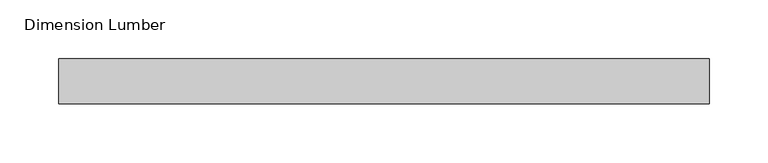
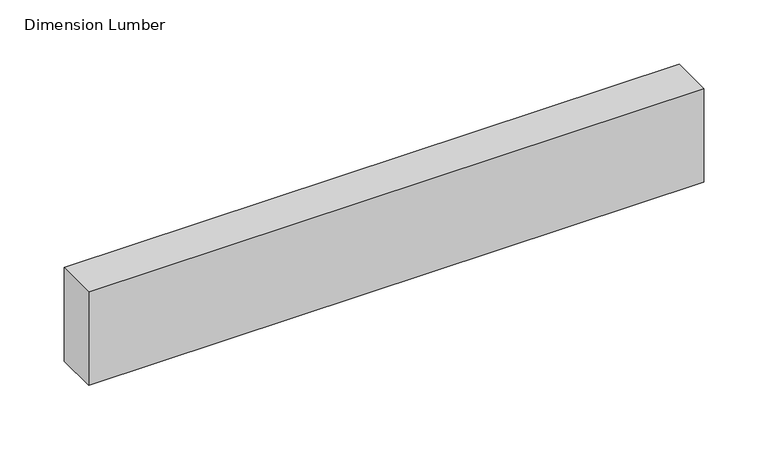
"""IFC4 building model written with IfcOpenShell, lengths in millimetres: beam geometry, Dimension Lumber : Roof Lumbers."""

import ifcopenshell
import ifcopenshell.guid

model = None  # the IFC model being written
_history = None  # IfcOwnerHistory: only IFC2X3 demands one
_inside = {}  # id of a spatial element -> (the spatial element, [elements in it])
_under = {}  # id of a project, library or spatial element -> (it, [spatial elements below it])
_declared = {}  # id of a project -> (the project, [libraries it declares])
_typed = {}  # id of a type object -> (the type object, [elements of that type])
_made_of = {}  # id of a material, layer set ... -> (it, [elements and type objects made of it])


def new_model(schema):
    """Start an empty IFC model of exactly this schema.

    Asked for "IFC4X3", IfcOpenShell would pick the latest addendum, in which some entities
    have other attributes; the version numbers below select the first issue.
    IFC2X3 requires an IfcOwnerHistory on every rooted entity: one is made here for all.
    """
    global model, _history
    if schema == "IFC4X3":
        model = ifcopenshell.file(schema_version=(4, 3, 0, 0))
    else:
        model = ifcopenshell.file(schema=schema)
    _inside.clear()
    _under.clear()
    _declared.clear()
    _typed.clear()
    _made_of.clear()
    _history = None
    if model.schema == "IFC2X3":
        org = make("IfcOrganization", Name="unknown")
        user = make(
            "IfcPersonAndOrganization",
            ThePerson=make("IfcPerson", FamilyName="unknown"),
            TheOrganization=org,
        )
        app = make(
            "IfcApplication",
            ApplicationDeveloper=org,
            Version="unknown",
            ApplicationFullName="unknown",
            ApplicationIdentifier="unknown",
        )
        _history = make(
            "IfcOwnerHistory",
            OwningUser=user,
            OwningApplication=app,
            ChangeAction="ADDED",
            CreationDate=0,
        )
    return model


def make(cls, **values):
    """One entity of the class cls with the attributes given. An attribute that is None is left unset."""
    return model.create_entity(
        cls, **{name: value for name, value in values.items() if value is not None}
    )


def rooted(cls, **values):
    """An entity with a GlobalId (a new one), such as an element, a storey or a relation."""
    return make(cls, GlobalId=ifcopenshell.guid.new(), OwnerHistory=_history, **values)


def si_unit(unit_type, name, prefix=None):
    """IfcSIUnit, for example si_unit("LENGTHUNIT", "METRE", prefix="MILLI")."""
    return make("IfcSIUnit", UnitType=unit_type, Prefix=prefix, Name=name)


def assignment(units):
    """IfcUnitAssignment: the units of a project."""
    return None if units is None else make("IfcUnitAssignment", Units=units)


def point(xyz):
    """IfcCartesianPoint."""
    return None if xyz is None else make("IfcCartesianPoint", Coordinates=xyz)


def direction(xyz):
    """IfcDirection."""
    return None if xyz is None else make("IfcDirection", DirectionRatios=xyz)


def frame(location, z_axis=None, x_axis=None):
    """IfcAxis2Placement3D, a coordinate frame: its origin and axes. An axis left out is left unset."""
    return make(
        "IfcAxis2Placement3D",
        Location=point(location),
        Axis=direction(z_axis),
        RefDirection=direction(x_axis),
    )


def origin():
    """The frame at (0, 0, 0) with its axes left unset."""
    return frame((0.0, 0.0, 0.0))


def place(relative_to, where):
    """IfcLocalPlacement: puts the frame where relative to a parent placement (None: the world)."""
    return make(
        "IfcLocalPlacement", PlacementRelTo=relative_to, RelativePlacement=where
    )


def context(
    kind, dimensions, precision=None, world=None, true_north=None, identifier=None
):
    """IfcGeometricRepresentationContext, for example the 3D "Model" context."""
    return make(
        "IfcGeometricRepresentationContext",
        ContextIdentifier=identifier,
        ContextType=kind,
        CoordinateSpaceDimension=dimensions,
        Precision=precision,
        WorldCoordinateSystem=world,
        TrueNorth=true_north,
    )


def project(units=None, contexts=None):
    """IfcProject with its units and contexts."""
    return rooted(
        "IfcProject",
        Name="project",
        RepresentationContexts=contexts,
        UnitsInContext=assignment(units),
    )


def spatial(cls, under=None, at=None, **own):
    """A site, building, storey or space (cls), placed at a placement, below another one or the project."""
    s = rooted(cls, ObjectPlacement=at, **own)
    if under is not None:
        _under.setdefault(under.id(), (under, []))[1].append(s)
    return s


def polyline(points):
    """IfcPolyline through the points."""
    return make("IfcPolyline", Points=[point(p) for p in points])


def outline(outer, holes=None, kind="AREA"):
    """IfcArbitraryClosedProfileDef: a profile drawn as a closed curve; with holes, ...WithVoids."""
    if holes is None:
        return make("IfcArbitraryClosedProfileDef", ProfileType=kind, OuterCurve=outer)
    return make(
        "IfcArbitraryProfileDefWithVoids",
        ProfileType=kind,
        OuterCurve=outer,
        InnerCurves=holes,
    )


def extrude(swept, where, along, depth):
    """IfcExtrudedAreaSolid: the profile swept, set in the frame where, extruded along a direction by depth."""
    return make(
        "IfcExtrudedAreaSolid",
        SweptArea=swept,
        Position=where,
        ExtrudedDirection=direction(along),
        Depth=depth,
    )


def shape(context_of_items, identifier, shape_type, items):
    """IfcShapeRepresentation: the items that make up one representation, for example the "Body"."""
    return make(
        "IfcShapeRepresentation",
        ContextOfItems=context_of_items,
        RepresentationIdentifier=identifier,
        RepresentationType=shape_type,
        Items=items,
    )


def source(mapping_origin, context_of_items, identifier, shape_type, items):
    """IfcRepresentationMap: a shape defined once, which mapped items show again and again."""
    return make(
        "IfcRepresentationMap",
        MappingOrigin=mapping_origin,
        MappedRepresentation=shape(context_of_items, identifier, shape_type, items),
    )


def transform(
    local_origin,
    x_axis=None,
    y_axis=None,
    z_axis=None,
    scale=None,
    scale2=None,
    scale3=None,
    uniform=True,
):
    """IfcCartesianTransformationOperator3D, or its non-uniform kind. x_axis, y_axis, z_axis: its Axis1, 2, 3."""
    if uniform:
        return make(
            "IfcCartesianTransformationOperator3D",
            Axis1=direction(x_axis),
            Axis2=direction(y_axis),
            LocalOrigin=point(local_origin),
            Scale=scale,
            Axis3=direction(z_axis),
        )
    return make(
        "IfcCartesianTransformationOperator3DnonUniform",
        Axis1=direction(x_axis),
        Axis2=direction(y_axis),
        LocalOrigin=point(local_origin),
        Scale=scale,
        Axis3=direction(z_axis),
        Scale2=scale2,
        Scale3=scale3,
    )


def mapped(mapping_source, mapping_target):
    """IfcMappedItem: shows the shape of a source again, moved by a transform."""
    return make(
        "IfcMappedItem", MappingSource=mapping_source, MappingTarget=mapping_target
    )


def made_of(thing, what):
    """Note that an element or type object is made of a material, layer set ...; save() writes the relation."""
    if what is not None:
        _made_of.setdefault(what.id(), (what, []))[1].append(thing)
    return thing


def element(
    cls,
    number,
    at=None,
    inside=None,
    cuts=None,
    type_object=None,
    material=None,
    context=None,
    identifier="Body",
    shape_type=None,
    held_by="IfcProductDefinitionShape",
    body=None,
    shapes=None,
    **own,
):
    """One element of the class cls, such as IfcWall. Its Tag is "e" and its number.

    at: its placement. inside: the storey or other place that contains it. cuts: it is an
    opening in that element (IfcRelVoidsElement). A single representation is given by context,
    identifier, shape_type and body (its items); several are given by shapes. held_by: the class
    of the entity that holds the representations. save() writes the other relations.
    """
    e = rooted(cls, Tag="e%d" % number, ObjectPlacement=at, **own)
    if body is not None:
        shapes = [shape(context, identifier, shape_type, body)]
    if shapes is not None:
        e.Representation = make(held_by, Representations=shapes)
    if inside is not None:
        _inside.setdefault(inside.id(), (inside, []))[1].append(e)
    if cuts is not None:
        rooted(
            "IfcRelVoidsElement", RelatingBuildingElement=cuts, RelatedOpeningElement=e
        )
    if type_object is not None:
        _typed.setdefault(type_object.id(), (type_object, []))[1].append(e)
    return made_of(e, material)


def aggregate(whole, parts):
    """IfcRelAggregates: a whole, such as a stair, and the parts it consists of."""
    return rooted("IfcRelAggregates", RelatingObject=whole, RelatedObjects=parts)


def save(model, path):
    """Write the relations noted so far, then the file.

    IfcRelAggregates (storeys below a building ...), IfcRelContainedInSpatialStructure (elements
    in a storey), IfcRelDefinesByType, IfcRelAssociatesMaterial and IfcRelDeclares: one each for
    every whole, place, type object, material and project.
    """
    for whole, parts in _under.values():
        aggregate(whole, parts)
    for where, things in _inside.values():
        rooted(
            "IfcRelContainedInSpatialStructure",
            RelatedElements=things,
            RelatingStructure=where,
        )
    for kind, things in _typed.values():
        rooted("IfcRelDefinesByType", RelatedObjects=things, RelatingType=kind)
    for what, things in _made_of.values():
        rooted("IfcRelAssociatesMaterial", RelatedObjects=things, RelatingMaterial=what)
    for by, libraries in _declared.values():
        rooted("IfcRelDeclares", RelatingContext=by, RelatedDefinitions=libraries)
    model.write(path)


def dimension_lumber_26660400(model_context):
    return source(origin(), model_context, "Body", "SweptSolid", [
        extrude(outline(polyline([(276.225, 19.05), (276.225, -19.05), (-276.225, -19.05), (-276.225, 19.05), (276.225, 19.05)])), frame((0.0, 0.0, -44.45), z_axis=(0.0, 0.0, 1.0), x_axis=(1.0, 0.0, 0.0)), (0.0, 0.0, 1.0), 88.9),
    ])


if __name__ == "__main__":
    model = new_model("IFC4")
    model_context = context("Model", 3, world=origin())
    ifc_project = project(units=[si_unit("LENGTHUNIT", "METRE", prefix="MILLI")], contexts=[model_context])
    site = spatial("IfcSite", under=ifc_project)
    building = spatial("IfcBuilding", under=site)
    placement = place(None, origin())
    dimension_lumber_shape = dimension_lumber_26660400(model_context)
    element("IfcBeam", 1, ObjectType="Dimension Lumber : Roof Lumbers", at=placement, inside=building, context=model_context, shape_type="MappedRepresentation", body=[
        mapped(dimension_lumber_shape, transform((0.0, 0.0, 0.0), x_axis=(1.0, 0.0, 0.0), y_axis=(0.0, 1.0, 0.0), z_axis=(0.0, 0.0, 1.0))),
    ])
    save(model, "model.ifc")

# Revit data of these elements
# Type "Dimension Lumber : Roof Lumbers"
#   Assembly Code = "B10"
#   A = 0.0364583 SF
#   Length [instance default] = 5' - 0"
#   b = 0' - 1 1/2"
#   d = 0' - 3 1/2"
#   Structural Material [instance default] = Softwood, Lumber
# Element 1 (IfcBeam, "Dimension Lumber : Roof Lumbers")
#   Structural Material = Douglas Fir #2
#   Materials on its faces: "Douglas Fir #2"
# Materials
#   "Softwood, Lumber": class "Wood", colour RGB 223 192 134, transparency 0, Description = "Pinus Echinata", Cost = 0
#   "Douglas Fir #2": class "Wood", colour RGB 223 192 134, transparency 0, Description = "Pinus Echinata", Cost = 0
